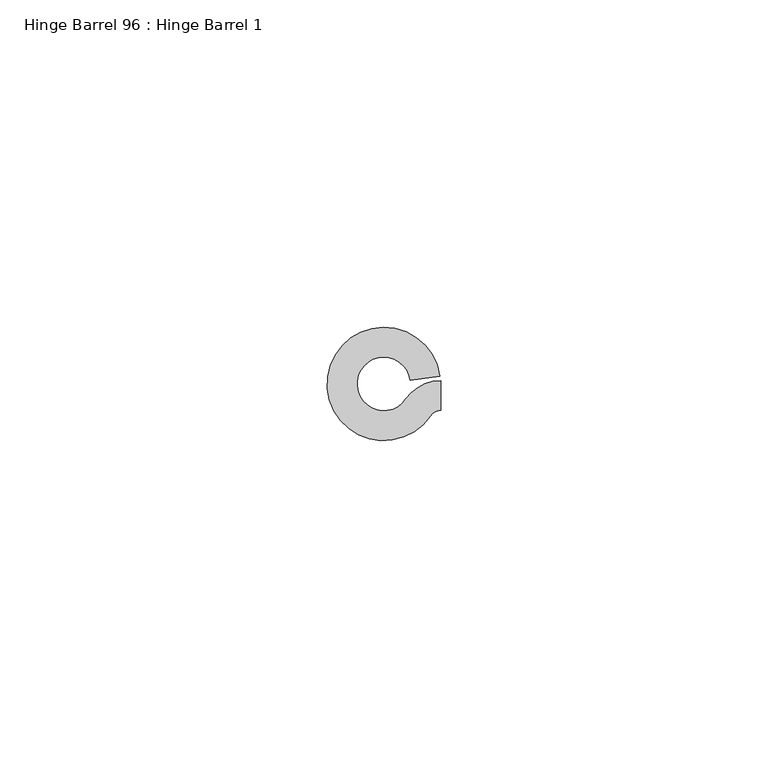
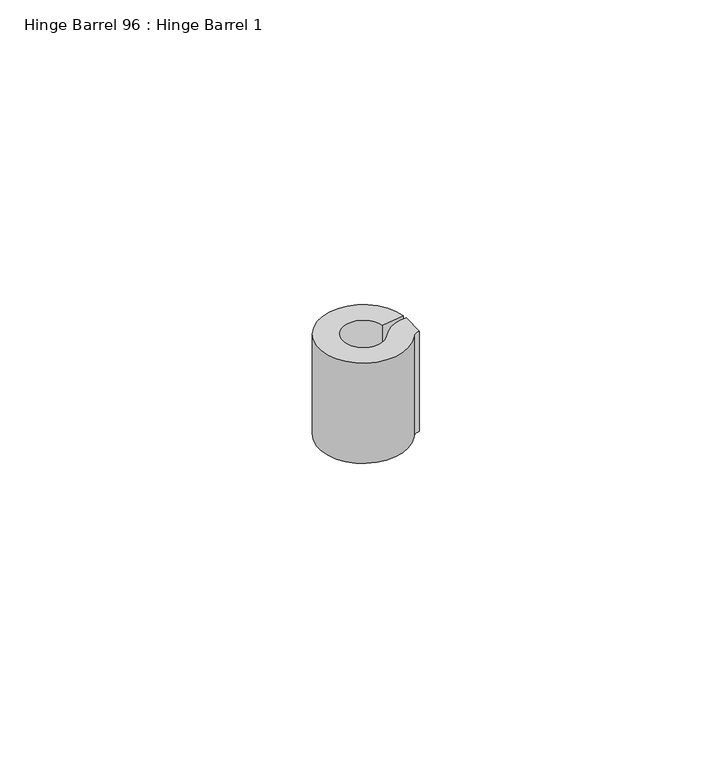
"""IFC4 building model written with IfcOpenShell, lengths in millimetres: proxy geometry, Hinge Barrel 96 : Hinge Barrel 1."""

from ifc_helpers import new_model, si_unit, point, frame, frame_2d, origin, place, context, project, spatial, polyline, circle_curve, trimmed, segment, composite_curve, outline, extrude, source, transform, mapped, element, save


def hinge_barrel_96_hinge_barrel_1_c85a10a0(model_context):
    return source(origin(), model_context, "Body", "SweptSolid", [
        extrude(outline(composite_curve([segment(trimmed(circle_curve(frame_2d((587327.8245257, -533990.5568067)), 6.4044851), [point((587322.5194669, -533986.9688017))], [point((587327.8245257, -533984.1523216))], False, "CARTESIAN"), True, "CONTINUOUS"), segment(polyline([(587327.8245257, -533984.1523216), (587327.8245257, -533988.7163841)]), True, "CONTINUOUS"), segment(trimmed(circle_curve(frame_2d((587327.8245257, -533990.5568067)), 1.8404226), [point((587327.8245257, -533988.7163841))], [point((587326.3000393, -533989.5257409))], True, "CARTESIAN"), True, "CONTINUOUS"), segment(trimmed(circle_curve(frame_2d((587319.1320739, -533984.6777841)), 8.6534625), [point((587326.3000393, -533989.5257409))], [point((587327.7022899, -533983.4803654))], False, "CARTESIAN"), True, "CONTINUOUS"), segment(polyline([(587327.7022899, -533983.4803654), (587323.1821338, -533984.1119153)]), True, "CONTINUOUS"), segment(trimmed(circle_curve(frame_2d((587319.1320739, -533984.6777841)), 4.0894), [point((587323.1821338, -533984.1119153))], [point((587322.5194669, -533986.9688017))], True, "CARTESIAN"), True, "CONTINUOUS")], self_intersect=False)), frame((0.0, 0.0, 438.15), z_axis=(0.0, 0.0, 1.0), x_axis=(1.0, 0.0, 0.0)), (0.0, 0.0, 1.0), 20.8359375),
    ])


if __name__ == "__main__":
    model = new_model("IFC4")
    model_context = context("Model", 3, world=origin())
    ifc_project = project(units=[si_unit("LENGTHUNIT", "METRE", prefix="MILLI")], contexts=[model_context])
    site = spatial("IfcSite", under=ifc_project)
    building = spatial("IfcBuilding", under=site)
    placement = place(None, origin())
    hinge_barrel_96_hinge_barrel_1_shape = hinge_barrel_96_hinge_barrel_1_c85a10a0(model_context)
    element("IfcBuildingElementProxy", 1, Name="Hinge Barrel 96 : Hinge Barrel 1", ObjectType="Hinge Barrel 96 : Hinge Barrel 1", at=placement, inside=building, context=model_context, shape_type="MappedRepresentation", body=[
        mapped(hinge_barrel_96_hinge_barrel_1_shape, transform((0.0, 0.0, 0.0), x_axis=(1.0, 0.0, 0.0), y_axis=(0.0, 1.0, 0.0), z_axis=(0.0, 0.0, 1.0))),
    ])
    save(model, "model.ifc")

# Revit data of these elements
# Element 1 (IfcBuildingElementProxy, "Hinge Barrel 96 : Hinge Barrel 1")
#   Materials on its faces: "6\"X6\" WELD-ON STL BUTT HINGE"
# Materials
#   "6\"X6\" WELD-ON STL BUTT HINGE": class "Metal", colour RGB 189 187 185, transparency 0, Description = "Carbon steel", Cost = 0
